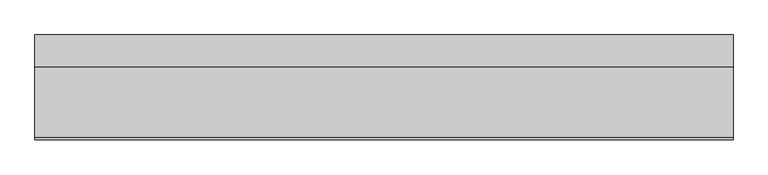
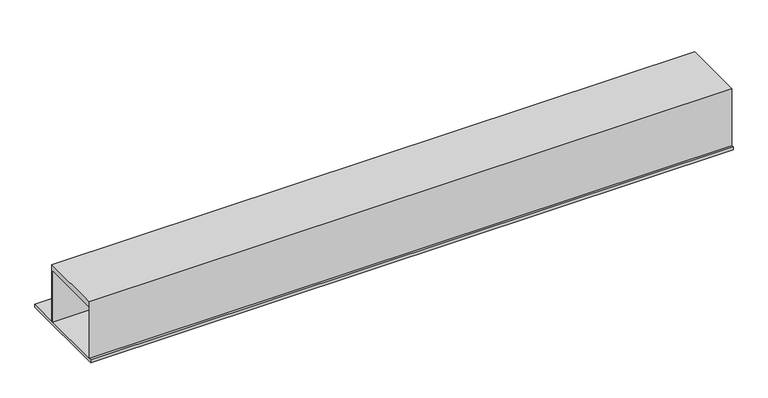
"""IFC4 building model written with IfcOpenShell, lengths in millimetres: beam geometry, NLRS_28_SF_LIB_stalen ligger THQ-AV-CWV-MMBS-SRP_gen_rsf : stalen ligger_gen__PET 280x6-290x30-450x15."""

import ifcopenshell
import ifcopenshell.guid

model = None  # the IFC model being written
_history = None  # IfcOwnerHistory: only IFC2X3 demands one
_inside = {}  # id of a spatial element -> (the spatial element, [elements in it])
_under = {}  # id of a project, library or spatial element -> (it, [spatial elements below it])
_declared = {}  # id of a project -> (the project, [libraries it declares])
_typed = {}  # id of a type object -> (the type object, [elements of that type])
_made_of = {}  # id of a material, layer set ... -> (it, [elements and type objects made of it])


def new_model(schema):
    """Start an empty IFC model of exactly this schema.

    Asked for "IFC4X3", IfcOpenShell would pick the latest addendum, in which some entities
    have other attributes; the version numbers below select the first issue.
    IFC2X3 requires an IfcOwnerHistory on every rooted entity: one is made here for all.
    """
    global model, _history
    if schema == "IFC4X3":
        model = ifcopenshell.file(schema_version=(4, 3, 0, 0))
    else:
        model = ifcopenshell.file(schema=schema)
    _inside.clear()
    _under.clear()
    _declared.clear()
    _typed.clear()
    _made_of.clear()
    _history = None
    if model.schema == "IFC2X3":
        org = make("IfcOrganization", Name="unknown")
        user = make(
            "IfcPersonAndOrganization",
            ThePerson=make("IfcPerson", FamilyName="unknown"),
            TheOrganization=org,
        )
        app = make(
            "IfcApplication",
            ApplicationDeveloper=org,
            Version="unknown",
            ApplicationFullName="unknown",
            ApplicationIdentifier="unknown",
        )
        _history = make(
            "IfcOwnerHistory",
            OwningUser=user,
            OwningApplication=app,
            ChangeAction="ADDED",
            CreationDate=0,
        )
    return model


def make(cls, **values):
    """One entity of the class cls with the attributes given. An attribute that is None is left unset."""
    return model.create_entity(
        cls, **{name: value for name, value in values.items() if value is not None}
    )


def rooted(cls, **values):
    """An entity with a GlobalId (a new one), such as an element, a storey or a relation."""
    return make(cls, GlobalId=ifcopenshell.guid.new(), OwnerHistory=_history, **values)


def si_unit(unit_type, name, prefix=None):
    """IfcSIUnit, for example si_unit("LENGTHUNIT", "METRE", prefix="MILLI")."""
    return make("IfcSIUnit", UnitType=unit_type, Prefix=prefix, Name=name)


def assignment(units):
    """IfcUnitAssignment: the units of a project."""
    return None if units is None else make("IfcUnitAssignment", Units=units)


def point(xyz):
    """IfcCartesianPoint."""
    return None if xyz is None else make("IfcCartesianPoint", Coordinates=xyz)


def direction(xyz):
    """IfcDirection."""
    return None if xyz is None else make("IfcDirection", DirectionRatios=xyz)


def frame(location, z_axis=None, x_axis=None):
    """IfcAxis2Placement3D, a coordinate frame: its origin and axes. An axis left out is left unset."""
    return make(
        "IfcAxis2Placement3D",
        Location=point(location),
        Axis=direction(z_axis),
        RefDirection=direction(x_axis),
    )


def origin():
    """The frame at (0, 0, 0) with its axes left unset."""
    return frame((0.0, 0.0, 0.0))


def place(relative_to, where):
    """IfcLocalPlacement: puts the frame where relative to a parent placement (None: the world)."""
    return make(
        "IfcLocalPlacement", PlacementRelTo=relative_to, RelativePlacement=where
    )


def context(
    kind, dimensions, precision=None, world=None, true_north=None, identifier=None
):
    """IfcGeometricRepresentationContext, for example the 3D "Model" context."""
    return make(
        "IfcGeometricRepresentationContext",
        ContextIdentifier=identifier,
        ContextType=kind,
        CoordinateSpaceDimension=dimensions,
        Precision=precision,
        WorldCoordinateSystem=world,
        TrueNorth=true_north,
    )


def project(units=None, contexts=None):
    """IfcProject with its units and contexts."""
    return rooted(
        "IfcProject",
        Name="project",
        RepresentationContexts=contexts,
        UnitsInContext=assignment(units),
    )


def spatial(cls, under=None, at=None, **own):
    """A site, building, storey or space (cls), placed at a placement, below another one or the project."""
    s = rooted(cls, ObjectPlacement=at, **own)
    if under is not None:
        _under.setdefault(under.id(), (under, []))[1].append(s)
    return s


def polyline(points):
    """IfcPolyline through the points."""
    return make("IfcPolyline", Points=[point(p) for p in points])


def outline(outer, holes=None, kind="AREA"):
    """IfcArbitraryClosedProfileDef: a profile drawn as a closed curve; with holes, ...WithVoids."""
    if holes is None:
        return make("IfcArbitraryClosedProfileDef", ProfileType=kind, OuterCurve=outer)
    return make(
        "IfcArbitraryProfileDefWithVoids",
        ProfileType=kind,
        OuterCurve=outer,
        InnerCurves=holes,
    )


def extrude(swept, where, along, depth):
    """IfcExtrudedAreaSolid: the profile swept, set in the frame where, extruded along a direction by depth."""
    return make(
        "IfcExtrudedAreaSolid",
        SweptArea=swept,
        Position=where,
        ExtrudedDirection=direction(along),
        Depth=depth,
    )


def shape(context_of_items, identifier, shape_type, items):
    """IfcShapeRepresentation: the items that make up one representation, for example the "Body"."""
    return make(
        "IfcShapeRepresentation",
        ContextOfItems=context_of_items,
        RepresentationIdentifier=identifier,
        RepresentationType=shape_type,
        Items=items,
    )


def source(mapping_origin, context_of_items, identifier, shape_type, items):
    """IfcRepresentationMap: a shape defined once, which mapped items show again and again."""
    return make(
        "IfcRepresentationMap",
        MappingOrigin=mapping_origin,
        MappedRepresentation=shape(context_of_items, identifier, shape_type, items),
    )


def transform(
    local_origin,
    x_axis=None,
    y_axis=None,
    z_axis=None,
    scale=None,
    scale2=None,
    scale3=None,
    uniform=True,
):
    """IfcCartesianTransformationOperator3D, or its non-uniform kind. x_axis, y_axis, z_axis: its Axis1, 2, 3."""
    if uniform:
        return make(
            "IfcCartesianTransformationOperator3D",
            Axis1=direction(x_axis),
            Axis2=direction(y_axis),
            LocalOrigin=point(local_origin),
            Scale=scale,
            Axis3=direction(z_axis),
        )
    return make(
        "IfcCartesianTransformationOperator3DnonUniform",
        Axis1=direction(x_axis),
        Axis2=direction(y_axis),
        LocalOrigin=point(local_origin),
        Scale=scale,
        Axis3=direction(z_axis),
        Scale2=scale2,
        Scale3=scale3,
    )


def mapped(mapping_source, mapping_target):
    """IfcMappedItem: shows the shape of a source again, moved by a transform."""
    return make(
        "IfcMappedItem", MappingSource=mapping_source, MappingTarget=mapping_target
    )


def made_of(thing, what):
    """Note that an element or type object is made of a material, layer set ...; save() writes the relation."""
    if what is not None:
        _made_of.setdefault(what.id(), (what, []))[1].append(thing)
    return thing


def element(
    cls,
    number,
    at=None,
    inside=None,
    cuts=None,
    type_object=None,
    material=None,
    context=None,
    identifier="Body",
    shape_type=None,
    held_by="IfcProductDefinitionShape",
    body=None,
    shapes=None,
    **own,
):
    """One element of the class cls, such as IfcWall. Its Tag is "e" and its number.

    at: its placement. inside: the storey or other place that contains it. cuts: it is an
    opening in that element (IfcRelVoidsElement). A single representation is given by context,
    identifier, shape_type and body (its items); several are given by shapes. held_by: the class
    of the entity that holds the representations. save() writes the other relations.
    """
    e = rooted(cls, Tag="e%d" % number, ObjectPlacement=at, **own)
    if body is not None:
        shapes = [shape(context, identifier, shape_type, body)]
    if shapes is not None:
        e.Representation = make(held_by, Representations=shapes)
    if inside is not None:
        _inside.setdefault(inside.id(), (inside, []))[1].append(e)
    if cuts is not None:
        rooted(
            "IfcRelVoidsElement", RelatingBuildingElement=cuts, RelatedOpeningElement=e
        )
    if type_object is not None:
        _typed.setdefault(type_object.id(), (type_object, []))[1].append(e)
    return made_of(e, material)


def aggregate(whole, parts):
    """IfcRelAggregates: a whole, such as a stair, and the parts it consists of."""
    return rooted("IfcRelAggregates", RelatingObject=whole, RelatedObjects=parts)


def save(model, path):
    """Write the relations noted so far, then the file.

    IfcRelAggregates (storeys below a building ...), IfcRelContainedInSpatialStructure (elements
    in a storey), IfcRelDefinesByType, IfcRelAssociatesMaterial and IfcRelDeclares: one each for
    every whole, place, type object, material and project.
    """
    for whole, parts in _under.values():
        aggregate(whole, parts)
    for where, things in _inside.values():
        rooted(
            "IfcRelContainedInSpatialStructure",
            RelatedElements=things,
            RelatingStructure=where,
        )
    for kind, things in _typed.values():
        rooted("IfcRelDefinesByType", RelatedObjects=things, RelatingType=kind)
    for what, things in _made_of.values():
        rooted("IfcRelAssociatesMaterial", RelatedObjects=things, RelatingMaterial=what)
    for by, libraries in _declared.values():
        rooted("IfcRelDeclares", RelatingContext=by, RelatedDefinitions=libraries)
    model.write(path)


def beam_7c9e214b(model_context):
    return source(origin(), model_context, "Body", "SweptSolid", [
        extrude(outline(polyline([(139.5, 280.0), (139.5, 0.0), (277.5, 0.0), (277.5, -15.0), (-172.5, -15.0), (-172.5, 0.0), (-162.5, 0.0), (-162.5, 280.0), (139.5, 280.0)]), holes=[polyline([(133.5, 0.0), (133.5, 250.0), (-156.5, 250.0), (-156.5, 0.0), (133.5, 0.0)])]), frame((-1499.9999994, 0.0, 0.0), z_axis=(1.0, 0.0, 0.0), x_axis=(0.0, 1.0, 0.0)), (0.0, 0.0, 1.0), 2999.9999988),
    ])


if __name__ == "__main__":
    model = new_model("IFC4")
    model_context = context("Model", 3, world=origin())
    ifc_project = project(units=[si_unit("LENGTHUNIT", "METRE", prefix="MILLI")], contexts=[model_context])
    site = spatial("IfcSite", under=ifc_project)
    building = spatial("IfcBuilding", under=site)
    placement = place(None, origin())
    beam_shape = beam_7c9e214b(model_context)
    element("IfcBeam", 1, ObjectType="NLRS_28_SF_LIB_stalen ligger THQ-AV-CWV-MMBS-SRP_gen_rsf : stalen ligger_gen__PET 280x6-290x30-450x15", at=placement, inside=building, context=model_context, shape_type="MappedRepresentation", body=[
        mapped(beam_shape, transform((0.0, 0.0, 0.0), x_axis=(1.0, 0.0, 0.0), y_axis=(0.0, 1.0, 0.0), z_axis=(0.0, 0.0, 1.0))),
    ])
    save(model, "model.ifc")

# Revit data of these elements
# Type "NLRS_28_SF_LIB_stalen ligger THQ-AV-CWV-MMBS-SRP_gen_rsf : stalen ligger_gen__PET 280x6-290x30-450x15"
#   Type IfcGUID = "0zo1UjqZ91lRsfCKsOOaAF"
#   IfcExportAs = "IfcBeamType"
#   Type Comments = "PET 280x6-290x30-450x15"
#   Model = " "
#   Manufacturer = " "
#   Fire Rating = " "
#   Description = "stalen ligger PET 280x6-290x30-450x15"
#   Assembly Code = "28.11"
#   tw = 6 mm
#   tu = 15 mm
#   to = 30 mm
#   h = 280 mm
#   bu = 450 mm
#   bo = 290 mm
#   NLRS_C_lengte [instance default] = 1500 mm
#   Length [instance default] = 1500 mm
#   RSF_C_vullen_met_beton [instance default] = no
#   RSF_C_petligger = yes
#   RSF_C_hoedligger = no
#   Structural Material = NLRS_h2_staal_gen_rsf
#   Keynote = ""
# Element 1 (IfcBeam, "NLRS_28_SF_LIB_stalen ligger THQ-AV-CWV-MMBS-SRP_gen_rsf : stalen ligger_gen__PET 280x6-290x30-450x15")
#   NLRS_C_lengte = 3000 mm
#   Materials on its faces: "NLRS_h2_staal_gen_rsf"
# Materials
#   "NLRS_h2_staal_gen_rsf": class "H - Metaal", colour RGB 189 187 185, transparency 0, Keynote = "h2", Manufacturer = "Revit Standards Foundation", URL = "www.revitstandards.org", Description = "staal", Cost = 0
